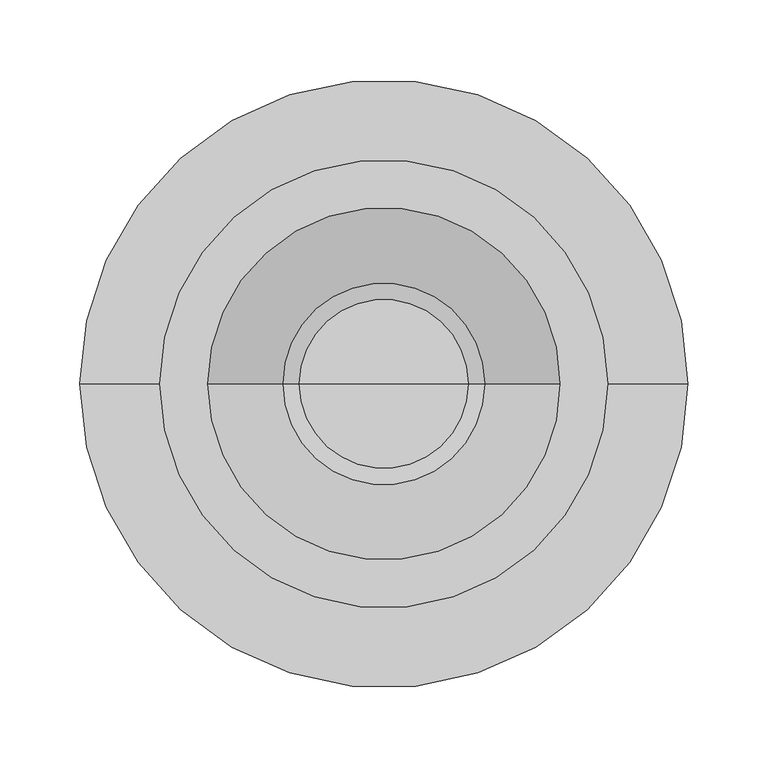
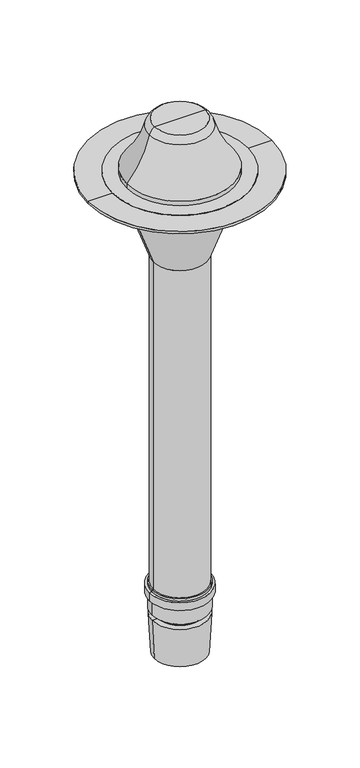
"""IFC4 building model written with IfcOpenShell, lengths in millimetres: proxy geometry, TN_Воронка ремонтная ТехноНИКОЛЬ PRO : Воронка ремонтная ТехноНИКОЛЬ PRO с листоуловителем 110x900 мм."""

from ifc_helpers import new_model, si_unit, point, frame, origin, origin_with_axes, origin_2d, place, context, project, spatial, polyline, circle_curve, ellipse_curve, trimmed, segment, composite_curve, outline, extrude, source, transform, mapped, element, save
from ifc_brep_helpers import plane_surface, cylinder_surface, revolved_surface, advanced_brep


def specialty_equipment_9ed86a26(model_context):
    return source(origin(), model_context, "Body", "SolidModel", [
        advanced_brep(
        [(57.9682619, 0.0, -900.0), (-57.9682619, 0.0, -900.0), (-57.9682619, 0.0, -895.0), (57.9682619, 0.0, -895.0), (62.9682619, 0.0, -900.0), (-62.9682619, 0.0, -900.0), (62.9682619, 0.0, -917.0324279), (-62.9682619, 0.0, -917.0324279), (57.9682619, 0.0, -917.0324279), (-57.9682619, 0.0, -917.0324279), (57.9682619, 0.0, -950.1985111), (-57.9682619, 0.0, -950.1985111), (44.9034904, 0.0, -960.7781544), (-44.9034904, 0.0, -960.7781544), (44.9034904, 0.0, -962.2889539), (-44.9034904, 0.0, -962.2889539), (57.3268553, 0.0, -962.2889539), (-57.3268553, 0.0, -962.2889539), (52.8873375, 0.0, -1047.0), (-52.8873375, 0.0, -1047.0), (41.9297278, 0.0, -1047.0), (-41.9297278, 0.0, -1047.0), (-54.9489754, 0.0, -895.0), (54.9489754, 0.0, -895.0), (41.9297278, 0.0, -958.7906616), (-41.9297278, 0.0, -958.7906616), (54.9489754, 0.0, -948.2478828), (-54.9489754, 0.0, -948.2478828)],
        [
            (0, 1, circle_curve(frame((0.0, 0.0, -900.0), z_axis=(0.0, 0.0, 1.0), x_axis=(-1.0, 0.0, 0.0)), 57.9682619)),
            (1, 2),
            (2, 3, circle_curve(frame((0.0, 0.0, -895.0), z_axis=(0.0, 0.0, -1.0), x_axis=(-1.0, 0.0, 0.0)), 57.9682619)),
            (3, 0),
            (1, 0, circle_curve(frame((0.0, 0.0, -900.0), z_axis=(0.0, 0.0, 1.0), x_axis=(-1.0, 0.0, 0.0)), 57.9682619)),
            (3, 2, circle_curve(frame((0.0, 0.0, -895.0), z_axis=(0.0, 0.0, -1.0), x_axis=(-1.0, 0.0, 0.0)), 57.9682619)),
            (4, 5, circle_curve(frame((0.0, 0.0, -900.0), z_axis=(0.0, 0.0, 1.0), x_axis=(-1.0, 0.0, 0.0)), 62.9682619)),
            (5, 1),
            (0, 4),
            (5, 4, circle_curve(frame((0.0, 0.0, -900.0), z_axis=(0.0, 0.0, 1.0), x_axis=(-1.0, 0.0, 0.0)), 62.9682619)),
            (6, 7, circle_curve(frame((0.0, 0.0, -917.0324279), z_axis=(0.0, 0.0, 1.0), x_axis=(-1.0, 0.0, 0.0)), 62.9682619)),
            (7, 5),
            (4, 6),
            (7, 6, circle_curve(frame((0.0, 0.0, -917.0324279), z_axis=(0.0, 0.0, 1.0), x_axis=(-1.0, 0.0, 0.0)), 62.9682619)),
            (8, 9, circle_curve(frame((0.0, 0.0, -917.0324279), z_axis=(0.0, 0.0, 1.0), x_axis=(-1.0, 0.0, 0.0)), 57.9682619)),
            (9, 7),
            (6, 8),
            (9, 8, circle_curve(frame((0.0, 0.0, -917.0324279), z_axis=(0.0, 0.0, 1.0), x_axis=(-1.0, 0.0, 0.0)), 57.9682619)),
            (10, 11, circle_curve(frame((0.0, 0.0, -950.1985111), z_axis=(0.0, 0.0, 1.0), x_axis=(-1.0, 0.0, 0.0)), 57.9682619)),
            (11, 9),
            (8, 10),
            (11, 10, circle_curve(frame((0.0, 0.0, -950.1985111), z_axis=(0.0, 0.0, 1.0), x_axis=(-1.0, 0.0, 0.0)), 57.9682619)),
            (12, 13, circle_curve(frame((0.0, 0.0, -960.7781544), z_axis=(0.0, 0.0, 1.0), x_axis=(-1.0, 0.0, 0.0)), 44.9034904)),
            (13, 11),
            (10, 12),
            (13, 12, circle_curve(frame((0.0, 0.0, -960.7781544), z_axis=(0.0, 0.0, 1.0), x_axis=(-1.0, 0.0, 0.0)), 44.9034904)),
            (14, 15, circle_curve(frame((0.0, 0.0, -962.2889539), z_axis=(0.0, 0.0, 1.0), x_axis=(-1.0, 0.0, 0.0)), 44.9034904)),
            (15, 13),
            (12, 14),
            (15, 14, circle_curve(frame((0.0, 0.0, -962.2889539), z_axis=(0.0, 0.0, 1.0), x_axis=(-1.0, 0.0, 0.0)), 44.9034904)),
            (16, 17, circle_curve(frame((0.0, 0.0, -962.2889539), z_axis=(0.0, 0.0, 1.0), x_axis=(-1.0, 0.0, 0.0)), 57.3268553)),
            (17, 15),
            (14, 16),
            (17, 16, circle_curve(frame((0.0, 0.0, -962.2889539), z_axis=(0.0, 0.0, 1.0), x_axis=(-1.0, 0.0, 0.0)), 57.3268553)),
            (18, 19, circle_curve(frame((0.0, 0.0, -1047.0), z_axis=(0.0, 0.0, 1.0), x_axis=(-1.0, 0.0, 0.0)), 52.8873375)),
            (19, 17),
            (16, 18),
            (19, 18, circle_curve(frame((0.0, 0.0, -1047.0), z_axis=(0.0, 0.0, 1.0), x_axis=(-1.0, 0.0, 0.0)), 52.8873375)),
            (20, 21, circle_curve(frame((0.0, 0.0, -1047.0), z_axis=(0.0, 0.0, 1.0), x_axis=(-1.0, 0.0, 0.0)), 41.9297278)),
            (21, 19),
            (18, 20),
            (21, 20, circle_curve(frame((0.0, 0.0, -1047.0), z_axis=(0.0, 0.0, 1.0), x_axis=(-1.0, 0.0, 0.0)), 41.9297278)),
            (2, 22),
            (22, 23, circle_curve(frame((0.0, 0.0, -895.0), z_axis=(0.0, 0.0, -1.0), x_axis=(-1.0, 0.0, 0.0)), 54.9489754)),
            (23, 3),
            (23, 22, circle_curve(frame((0.0, 0.0, -895.0), z_axis=(0.0, 0.0, -1.0), x_axis=(-1.0, 0.0, 0.0)), 54.9489754)),
            (24, 25, circle_curve(frame((0.0, 0.0, -958.7906616), z_axis=(0.0, 0.0, 1.0), x_axis=(-1.0, 0.0, 0.0)), 41.9297278)),
            (25, 21),
            (20, 24),
            (25, 24, circle_curve(frame((0.0, 0.0, -958.7906616), z_axis=(0.0, 0.0, 1.0), x_axis=(-1.0, 0.0, 0.0)), 41.9297278)),
            (26, 27, circle_curve(frame((0.0, 0.0, -948.2478828), z_axis=(0.0, 0.0, 1.0), x_axis=(-1.0, 0.0, 0.0)), 54.9489754)),
            (27, 25),
            (24, 26),
            (27, 26, circle_curve(frame((0.0, 0.0, -948.2478828), z_axis=(0.0, 0.0, 1.0), x_axis=(-1.0, 0.0, 0.0)), 54.9489754)),
            (22, 27),
            (26, 23),
        ],
        [
            cylinder_surface(frame((0.0, 0.0, 1167.3150031), z_axis=(0.0, 0.0, -1.0), x_axis=(-1.0, 0.0, 0.0)), 57.9682619),
            plane_surface(frame((0.0, 0.0, -900.0), z_axis=(0.0, 0.0, 1.0), x_axis=(-1.0, 0.0, 0.0))),
            cylinder_surface(frame((0.0, 0.0, 1167.3150031), z_axis=(0.0, 0.0, -1.0), x_axis=(-1.0, 0.0, 0.0)), 62.9682619),
            plane_surface(frame((0.0, 0.0, -917.0324279), z_axis=(0.0, 0.0, -1.0), x_axis=(-1.0, 0.0, 0.0))),
            revolved_surface(polyline([(-57.9682619, 0.0, -950.1985111), (-44.9034904, 0.0, -960.7781544)]), (0.0, 0.0, 1167.3150031), (0.0, 0.0, -1.0)),
            cylinder_surface(frame((0.0, 0.0, 1167.3150031), z_axis=(0.0, 0.0, -1.0), x_axis=(-1.0, 0.0, 0.0)), 44.9034904),
            plane_surface(frame((0.0, 0.0, -962.2889539), z_axis=(0.0, 0.0, 1.0), x_axis=(-1.0, 0.0, 0.0))),
            revolved_surface(polyline([(-57.3268553, 0.0, -962.2889539), (-52.8873375, 0.0, -1047.0)]), (0.0, 0.0, 1167.3150031), (0.0, 0.0, -1.0)),
            plane_surface(frame((0.0, 0.0, -1047.0), z_axis=(0.0, 0.0, -1.0), x_axis=(-1.0, 0.0, 0.0))),
            plane_surface(frame((0.0, 0.0, -895.0), z_axis=(0.0, 0.0, 1.0), x_axis=(-1.0, 0.0, 0.0))),
            revolved_surface(polyline([(-41.9297278, 0.0, -1047.0), (-41.9297278, 0.0, -958.7906616)]), (0.0, 0.0, 1167.3150031), (0.0, 0.0, -1.0)),
            revolved_surface(polyline([(-41.9297278, 0.0, -958.7906616), (-54.9489754, 0.0, -948.2478828)]), (0.0, 0.0, 1167.3150031), (0.0, 0.0, -1.0)),
            revolved_surface(polyline([(-54.9489754, 0.0, -948.2478827999998), (-54.9489754, 0.0, -895.0)]), (0.0, 0.0, 1167.3150031), (0.0, 0.0, -1.0)),
        ],
        [
            (0, [[1, 2, 3, 4]]),
            (0, [[5, -4, 6, -2]]),
            (1, [[7, 8, -1, 9]]),
            (1, [[10, -9, -5, -8]]),
            (2, [[11, 12, -7, 13]]),
            (2, [[14, -13, -10, -12]]),
            (3, [[15, 16, -11, 17]]),
            (3, [[18, -17, -14, -16]]),
            (0, [[19, 20, -15, 21]]),
            (0, [[22, -21, -18, -20]]),
            (4, [[23, 24, -19, 25]]),
            (4, [[26, -25, -22, -24]]),
            (5, [[27, 28, -23, 29]]),
            (5, [[30, -29, -26, -28]]),
            (6, [[31, 32, -27, 33]]),
            (6, [[34, -33, -30, -32]]),
            (7, [[35, 36, -31, 37]]),
            (7, [[38, -37, -34, -36]]),
            (8, [[39, 40, -35, 41]]),
            (8, [[42, -41, -38, -40]]),
            (9, [[-3, 43, 44, 45]]),
            (9, [[-6, -45, 46, -43]]),
            (10, [[47, 48, -39, 49]]),
            (10, [[50, -49, -42, -48]]),
            (11, [[51, 52, -47, 53]]),
            (11, [[54, -53, -50, -52]]),
            (12, [[-44, 55, -51, 56]]),
            (12, [[-46, -56, -54, -55]]),
        ],
    ),
        advanced_brep(
        [(110.0556416, 0.0, 0.0), (-110.0556416, 0.0, 0.0), (-110.0556416, 0.0, 10.0), (110.0556416, 0.0, 10.0), (0.0, 0.0, 0.0), (52.7728393, 0.0, 115.0), (-52.7728393, 0.0, 115.0), (0.0, 0.0, 115.0), (62.9807579, 0.0, 100.6532382), (-62.9807579, 0.0, 100.6532382)],
        [
            (0, 1, circle_curve(frame((0.0, 0.0, 0.0), z_axis=(0.0, 0.0, 1.0), x_axis=(-1.0, 0.0, 0.0)), 110.0556416)),
            (1, 2),
            (2, 3, circle_curve(frame((0.0, 0.0, 10.0), z_axis=(0.0, 0.0, -1.0), x_axis=(-1.0, 0.0, 0.0)), 110.0556416)),
            (3, 0),
            (1, 0, circle_curve(frame((0.0, 0.0, 0.0), z_axis=(0.0, 0.0, 1.0), x_axis=(-1.0, 0.0, 0.0)), 110.0556416)),
            (3, 2, circle_curve(frame((0.0, 0.0, 10.0), z_axis=(0.0, 0.0, -1.0), x_axis=(-1.0, 0.0, 0.0)), 110.0556416)),
            (4, 1),
            (0, 4),
            (5, 6, circle_curve(frame((0.0, 0.0, 115.0), z_axis=(0.0, 0.0, 1.0), x_axis=(-1.0, 0.0, 0.0)), 52.7728393)),
            (6, 7),
            (7, 5),
            (6, 5, circle_curve(frame((0.0, 0.0, 115.0), z_axis=(0.0, 0.0, 1.0), x_axis=(-1.0, 0.0, 0.0)), 52.7728393)),
            (8, 9, circle_curve(frame((0.0, 0.0, 100.6532382), z_axis=(0.0, 0.0, 1.0), x_axis=(-1.0, 0.0, 0.0)), 62.9807579)),
            (9, 6, circle_curve(frame((-39.8885443, 0.0, 95.0277285), z_axis=(0.0, 1.0, 0.0), x_axis=(1.0, 0.0, 0.0)), 23.7675553)),
            (5, 8, circle_curve(frame((39.8885443, 0.0, 95.0277285), z_axis=(0.0, 1.0, 0.0), x_axis=(-1.0, 0.0, 0.0)), 23.7675553)),
            (9, 8, circle_curve(frame((0.0, 0.0, 100.6532382), z_axis=(0.0, 0.0, 1.0), x_axis=(-1.0, 0.0, 0.0)), 62.9807579)),
            (2, 9, circle_curve(frame((-271.7387744, 0.0, 151.5089197), z_axis=(0.0, -1.0, 0.0), x_axis=(1.0, 0.0, 0.0)), 214.8632351)),
            (8, 3, circle_curve(frame((271.7387744, 0.0, 151.5089197), z_axis=(0.0, -1.0, 0.0), x_axis=(-1.0, 0.0, 0.0)), 214.8632351)),
        ],
        [
            cylinder_surface(frame((0.0, 0.0, 0.0), z_axis=(0.0, 0.0, -1.0), x_axis=(-1.0, 0.0, 0.0)), 110.0556416),
            plane_surface(frame((0.0, 0.0, 0.0), z_axis=(0.0, 0.0, -1.0), x_axis=(-1.0, 0.0, 0.0))),
            plane_surface(frame((0.0, 0.0, 115.0), z_axis=(0.0, 0.0, 1.0), x_axis=(-1.0, 0.0, 0.0))),
            revolved_surface(trimmed(ellipse_curve(frame((-39.8885443, 0.0, 95.0277285), z_axis=(0.0, -1.0, 0.0), x_axis=(1.0, 0.0, 0.0)), 23.7675553, 23.7675553), [point((-52.7728393, 0.0, 115.0))], [point((-62.9807579, 0.0, 100.6532382))], True, "CARTESIAN"), (0.0, 0.0, 0.0), (0.0, 0.0, -1.0)),
            revolved_surface(trimmed(ellipse_curve(frame((-271.7387744, 0.0, 151.5089197), z_axis=(0.0, 1.0, 0.0), x_axis=(1.0, 0.0, 0.0)), 214.8632351, 214.8632351), [point((-62.9807579, 0.0, 100.6532382))], [point((-110.0556416, 0.0, 10.0))], True, "CARTESIAN"), (0.0, 0.0, 0.0), (0.0, 0.0, -1.0)),
        ],
        [
            (0, [[1, 2, 3, 4]]),
            (0, [[5, -4, 6, -2]]),
            (1, [[7, -1, 8]]),
            (1, [[-8, -5, -7]]),
            (2, [[9, 10, 11]]),
            (2, [[12, -11, -10]]),
            (3, [[13, 14, -9, 15]]),
            (3, [[16, -15, -12, -14]]),
            (4, [[-3, 17, -13, 18]]),
            (4, [[-6, -18, -16, -17]]),
        ],
    ),
        extrude(outline(composite_curve([segment(trimmed(circle_curve(origin_2d(), 140.0), [point((-140.0, 0.0))], [point((140.0, 0.0))], False, "CARTESIAN"), True, "CONTINUOUS"), segment(trimmed(circle_curve(origin_2d(), 140.0), [point((140.0, 0.0))], [point((-140.0, 0.0))], False, "CARTESIAN"), True, "CONTINUOUS")], self_intersect=False), holes=[composite_curve([segment(trimmed(circle_curve(origin_2d(), 110.0556416), [point((-110.0556416, 0.0))], [point((110.0556416, 0.0))], True, "CARTESIAN"), True, "CONTINUOUS"), segment(trimmed(circle_curve(origin_2d(), 110.0556416), [point((110.0556416, 0.0))], [point((-110.0556416, 0.0))], True, "CARTESIAN"), True, "CONTINUOUS")], self_intersect=False)]), origin_with_axes(), (0.0, 0.0, 1.0), 1.0),
        advanced_brep(
        [(0.0, 0.0, -900.0), (-55.0, 0.0, -900.0), (55.0, 0.0, -900.0), (190.0, 0.0, 0.0), (-190.0, 0.0, 0.0), (-83.890873, 0.0, 0.0), (83.890873, 0.0, 0.0), (190.0, 0.0, -5.0), (-190.0, 0.0, -5.0), (93.890873, 0.0, -5.0), (-93.890873, 0.0, -5.0), (55.0, 0.0, -179.9935725), (-55.0, 0.0, -179.9935725), (-93.890873, 0.0, -71.109127), (93.890873, 0.0, -71.109127), (81.9669914, 0.0, -74.7632135), (-81.9669914, 0.0, -74.7632135), (0.0, 0.0, -74.7632135), (83.890873, 0.0, -69.3768397), (-83.890873, 0.0, -69.3768397)],
        [
            (0, 1),
            (1, 2, circle_curve(frame((0.0, 0.0, -900.0), z_axis=(0.0, 0.0, -1.0), x_axis=(-1.0, 0.0, 0.0)), 55.0)),
            (2, 0),
            (2, 1, circle_curve(frame((0.0, 0.0, -900.0), z_axis=(0.0, 0.0, -1.0), x_axis=(-1.0, 0.0, 0.0)), 55.0)),
            (3, 4, circle_curve(frame((0.0, 0.0, 0.0), z_axis=(0.0, 0.0, 1.0), x_axis=(-1.0, 0.0, 0.0)), 190.0)),
            (4, 5),
            (5, 6, circle_curve(frame((0.0, 0.0, 0.0), z_axis=(0.0, 0.0, -1.0), x_axis=(-1.0, 0.0, 0.0)), 83.890873)),
            (6, 3),
            (4, 3, circle_curve(frame((0.0, 0.0, 0.0), z_axis=(0.0, 0.0, 1.0), x_axis=(-1.0, 0.0, 0.0)), 190.0)),
            (6, 5, circle_curve(frame((0.0, 0.0, 0.0), z_axis=(0.0, 0.0, -1.0), x_axis=(-1.0, 0.0, 0.0)), 83.890873)),
            (7, 8, circle_curve(frame((0.0, 0.0, -5.0), z_axis=(0.0, 0.0, 1.0), x_axis=(-1.0, 0.0, 0.0)), 190.0)),
            (8, 4),
            (3, 7),
            (8, 7, circle_curve(frame((0.0, 0.0, -5.0), z_axis=(0.0, 0.0, 1.0), x_axis=(-1.0, 0.0, 0.0)), 190.0)),
            (9, 10, circle_curve(frame((0.0, 0.0, -5.0), z_axis=(0.0, 0.0, 1.0), x_axis=(-1.0, 0.0, 0.0)), 93.890873)),
            (10, 8),
            (7, 9),
            (10, 9, circle_curve(frame((0.0, 0.0, -5.0), z_axis=(0.0, 0.0, 1.0), x_axis=(-1.0, 0.0, 0.0)), 93.890873)),
            (11, 12, circle_curve(frame((0.0, 0.0, -179.9935725), z_axis=(0.0, 0.0, 1.0), x_axis=(-1.0, 0.0, 0.0)), 55.0)),
            (12, 13),
            (13, 14, circle_curve(frame((0.0, 0.0, -71.109127), z_axis=(0.0, 0.0, -1.0), x_axis=(-1.0, 0.0, 0.0)), 93.890873)),
            (14, 11),
            (12, 11, circle_curve(frame((0.0, 0.0, -179.9935725), z_axis=(0.0, 0.0, 1.0), x_axis=(-1.0, 0.0, 0.0)), 55.0)),
            (14, 13, circle_curve(frame((0.0, 0.0, -71.109127), z_axis=(0.0, 0.0, -1.0), x_axis=(-1.0, 0.0, 0.0)), 93.890873)),
            (1, 12),
            (11, 2),
            (15, 16, circle_curve(frame((0.0, 0.0, -74.7632135), z_axis=(0.0, 0.0, 1.0), x_axis=(-1.0, 0.0, 0.0)), 81.9669914)),
            (16, 17),
            (17, 15),
            (16, 15, circle_curve(frame((0.0, 0.0, -74.7632135), z_axis=(0.0, 0.0, 1.0), x_axis=(-1.0, 0.0, 0.0)), 81.9669914)),
            (18, 19, circle_curve(frame((0.0, 0.0, -69.3768397), z_axis=(0.0, 0.0, 1.0), x_axis=(-1.0, 0.0, 0.0)), 83.890873)),
            (19, 16),
            (15, 18),
            (19, 18, circle_curve(frame((0.0, 0.0, -69.3768397), z_axis=(0.0, 0.0, 1.0), x_axis=(-1.0, 0.0, 0.0)), 83.890873)),
            (5, 19),
            (18, 6),
            (13, 10),
            (9, 14),
        ],
        [
            plane_surface(frame((0.0, 0.0, -900.0), z_axis=(0.0, 0.0, -1.0), x_axis=(-1.0, 0.0, 0.0))),
            plane_surface(frame((0.0, 0.0, 0.0), z_axis=(0.0, 0.0, 1.0), x_axis=(-1.0, 0.0, 0.0))),
            cylinder_surface(frame((0.0, 0.0, 0.0), z_axis=(0.0, 0.0, -1.0), x_axis=(-1.0, 0.0, 0.0)), 190.0),
            plane_surface(frame((0.0, 0.0, -5.0), z_axis=(0.0, 0.0, -1.0), x_axis=(-1.0, 0.0, 0.0))),
            revolved_surface(polyline([(-93.890873, 0.0, -71.109127), (-55.0, 0.0, -179.9935725)]), (0.0, 0.0, 0.0), (0.0, 0.0, -1.0)),
            cylinder_surface(frame((0.0, 0.0, 0.0), z_axis=(0.0, 0.0, -1.0), x_axis=(-1.0, 0.0, 0.0)), 55.0),
            plane_surface(frame((0.0, 0.0, -74.7632135), z_axis=(0.0, 0.0, 1.0), x_axis=(-1.0, 0.0, 0.0))),
            revolved_surface(polyline([(-81.9669914, 0.0, -74.7632135), (-83.890873, 0.0, -69.3768397)]), (0.0, 0.0, 0.0), (0.0, 0.0, -1.0)),
            revolved_surface(polyline([(-83.890873, 0.0, -69.3768397), (-83.890873, 0.0, 0.0)]), (0.0, 0.0, 0.0), (0.0, 0.0, -1.0)),
            cylinder_surface(frame((0.0, 0.0, 0.0), z_axis=(0.0, 0.0, -1.0), x_axis=(-1.0, 0.0, 0.0)), 93.890873),
        ],
        [
            (0, [[1, 2, 3]]),
            (0, [[-3, 4, -1]]),
            (1, [[5, 6, 7, 8]]),
            (1, [[9, -8, 10, -6]]),
            (2, [[11, 12, -5, 13]]),
            (2, [[14, -13, -9, -12]]),
            (3, [[15, 16, -11, 17]]),
            (3, [[18, -17, -14, -16]]),
            (4, [[19, 20, 21, 22]]),
            (4, [[23, -22, 24, -20]]),
            (5, [[-2, 25, -19, 26]]),
            (5, [[-4, -26, -23, -25]]),
            (6, [[27, 28, 29]]),
            (6, [[30, -29, -28]]),
            (7, [[31, 32, -27, 33]]),
            (7, [[34, -33, -30, -32]]),
            (8, [[-7, 35, -31, 36]]),
            (8, [[-10, -36, -34, -35]]),
            (9, [[-21, 37, -15, 38]]),
            (9, [[-24, -38, -18, -37]]),
        ],
    ),
    ])


if __name__ == "__main__":
    model = new_model("IFC4")
    model_context = context("Model", 3, world=origin())
    ifc_project = project(units=[si_unit("LENGTHUNIT", "METRE", prefix="MILLI")], contexts=[model_context])
    site = spatial("IfcSite", under=ifc_project)
    building = spatial("IfcBuilding", under=site)
    placement = place(None, origin())
    specialty_equipment_shape = specialty_equipment_9ed86a26(model_context)
    element("IfcBuildingElementProxy", 1, Name="TN_Воронка ремонтная ТехноНИКОЛЬ PRO : Воронка ремонтная ТехноНИКОЛЬ PRO с листоуловителем 110x900 мм", ObjectType="TN_Воронка ремонтная ТехноНИКОЛЬ PRO : Воронка ремонтная ТехноНИКОЛЬ PRO с листоуловителем 110x900 мм", at=placement, inside=building, context=model_context, shape_type="MappedRepresentation", body=[
        mapped(specialty_equipment_shape, transform((0.0, 0.0, 0.0), x_axis=(1.0, 0.0, 0.0), y_axis=(0.0, 1.0, 0.0), z_axis=(0.0, 0.0, 1.0))),
    ])
    save(model, "model.ifc")

# Revit data of these elements
# Type "TN_Воронка ремонтная ТехноНИКОЛЬ PRO : Воронка ремонтная ТехноНИКОЛЬ PRO с листоуловителем 110x900 мм"
#   Description = "Кровельная ремонтная воронка применяется для быстрого монтажа в существующую магистраль водоотведения на кровле при проведении капитального ремонта. Воронка комплектуется листвоуловителем и обжимным фланцем из нержавеющей стали, без нагревательного элемента. Переходная муфта изготавливается из ПВХ. Применяется для соединения кровельных воронок ТехноНИКОЛЬ (диаметр патрубка 110 мм) с существующей ливневой канализацией на кровле с диаметром трубы 100 мм."
#   Manufacturer = "ТехноНИКОЛЬ"
#   URL = "https://www.tstn.ru/product/voronka-remontnaya-tekhnonikol-pro-s-listoulovitelem-110x900-mm-i-perekhodnoy-muftoy-90-110mm/"
#   ADSK_Примечание = ""
#   ADSK_Обозначение = "ТехноНИКОЛЬ"
#   ADSK_Наименование = "Воронка ремонтная ТехноНИКОЛЬ PRO с листоуловителем 110x900 мм"
#   ADSK_Масса_Текст = ""
#   ADSK_Марка = ""
#   ADSK_Код изделия = "659574"
#   ADSK_Завод-изготовитель = "ТехноНИКОЛЬ"
#   ADSK_Единица измерения = "шт."
#   ADSK_Группирование = "Комплектующие и воронки"
#   ADSK_URL страницы изделия = "https://www.tstn.ru/product/voronka-remontnaya-tekhnonikol-pro-s-listoulovitelem-110x900-mm-i-perekhodnoy-muftoy-90-110mm/"
#   ADSK_URL документации изделия = ""
#   Радиус = 55 mm
#   Отступ патрубка подключения [instance default] = 147 mm
#   Монтажный диаметр [instance default] = 90 mm
#   Длина расчетная [instance default] = 900 mm
#   Длина отвода [instance default] = 900 mm
#   ADSK_Количество = 1
#   Видимость_Муфта [instance default] = yes
#   Видимость_Листоуловитель [instance default] = yes
#   Материал_Фланец = TN_ПВХ_Серый
#   Материал_Корпус = TN_ПВХ_Черный
#   Default Elevation = 0
# Element 1 (IfcBuildingElementProxy, "TN_Воронка ремонтная ТехноНИКОЛЬ PRO : Воронка ремонтная ТехноНИКОЛЬ PRO с листоуловителем 110x900 мм")
#   Materials on its faces: "TN_ПВХ_Черный", "TN_ПВХ_Серый"
# Materials
#   "TN_ПВХ_Серый": class "Типовые", colour RGB 192 192 192, transparency 0, Cost = 0
#   "TN_ПВХ_Черный": class "Типовые", colour RGB 48 48 48, transparency 0, Cost = 0
